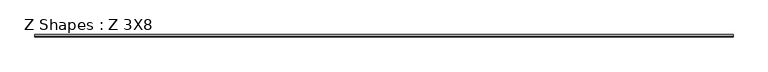
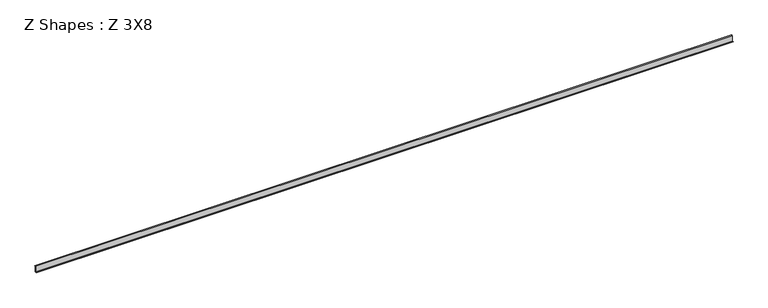
"""IFC4 building model written with IfcOpenShell, lengths in millimetres: beam geometry, Z Shapes : Z 3X8."""

from ifc_helpers import new_model, si_unit, frame, origin, place, context, project, spatial, polyline, outline, extrude, source, transform, mapped, element, save


def z_shapes_z_3x8_95925623(model_context):
    return source(origin(), model_context, "Body", "SweptSolid", [
        extrude(outline(polyline([(57.2805719, 92.452825), (27.1991352, 92.452825), (27.1991352, -98.809175), (-18.9194281, -98.809175), (-18.9194281, -92.459175), (19.1805719, -92.459175), (19.1805719, 102.104825), (57.2805719, 102.104825), (57.2805719, 92.452825)])), frame((-11671.3, 0.0, 0.0), z_axis=(1.0, 0.0, 0.0), x_axis=(0.0, 1.0, 0.0)), (0.0, 0.0, 1.0), 23342.6),
    ])


if __name__ == "__main__":
    model = new_model("IFC4")
    model_context = context("Model", 3, world=origin())
    ifc_project = project(units=[si_unit("LENGTHUNIT", "METRE", prefix="MILLI")], contexts=[model_context])
    site = spatial("IfcSite", under=ifc_project)
    building = spatial("IfcBuilding", under=site)
    placement = place(None, origin())
    z_shapes_z_3x8_shape = z_shapes_z_3x8_95925623(model_context)
    element("IfcBeam", 1, ObjectType="Z Shapes : Z 3X8", at=placement, inside=building, context=model_context, shape_type="MappedRepresentation", body=[
        mapped(z_shapes_z_3x8_shape, transform((0.0, 0.0, 0.0), x_axis=(1.0, 0.0, 0.0), y_axis=(0.0, 1.0, 0.0), z_axis=(0.0, 0.0, 1.0))),
    ])
    save(model, "model.ifc")

# Revit data of these elements
# Type "Z Shapes : Z 3X8"
#   Section Name Key = "W12x26"
#   Assembly Code = "B10"
#   Width = 76.2 mm
#   Web Thickness = 5.842 mm
#   Web Fillet = 7.62 mm
#   Warping Constant = 163001.3 cm⁶
#   Torsional Moment of Inertia = 12.4869 cm⁴
#   Section Area = 7.65 in²
#   Plastic Modulus weak axis = 0.00472801 (stored number, unit not read)
#   Plastic Modulus strong axis = 0.0215278 (stored number, unit not read)
#   Perimeter = 15.0571 m²/m
#   Nominal Weight = 379.441 N/m
#   Moment of Inertia weak axis = 720.08 cm⁴
#   Moment of Inertia strong axis = 8491.12 cm⁴
#   Height = 184.912 mm
#   Flange Thickness = 9.652 mm
#   Elastic Modulus weak axis = 0.00309028 (stored number, unit not read)
#   Elastic Modulus strong axis = 0.0193287 (stored number, unit not read)
#   Centroid Vertical = 92.456 mm
#   Centroid Horizontal = 38.1 mm
#   Length [instance default] = 5' - 0"
#   Structural Material [instance default] = Steel ASTM A992
#   Principal Axes Angle = 0
# Element 1 (IfcBeam, "Z Shapes : Z 3X8")
#   Structural Material = accent 2
#   Materials on its faces: "accent 2"
# Materials
#   "Steel ASTM A992": class "Metal", colour RGB 189 187 185, transparency 0, Description = "Structural steel 50ksi", Cost = 0
#   "accent 2": class "Wood", colour RGB 80 80 80, transparency 0, Description = "Wood framing, thermal airspace", Cost = 0
